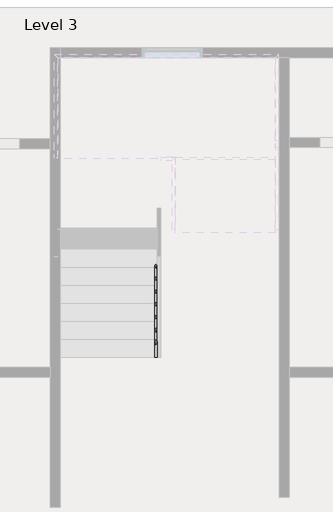
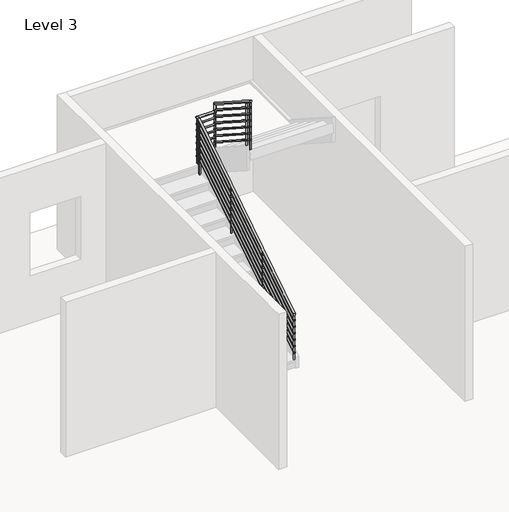
# One storey, part 6 of 7: 1 railing.
"""IFC4 building model written with IfcOpenShell, lengths in millimetres."""

from ifc_helpers import new_model, si_unit, point, frame, frame_2d, origin, place, context, project, spatial, circle_curve, ellipse_curve, trimmed, segment, composite_curve, outline, extrude, element, save
from ifc_brep_helpers import plane_surface, cylinder_surface, advanced_brep

model = new_model("IFC4")

# Units and contexts
model_context = context("Model", 3, world=origin())
ifc_project = project(units=[si_unit("LENGTHUNIT", "METRE", prefix="MILLI")], contexts=[model_context])

# Site, building, storey
site = spatial("IfcSite", under=ifc_project)
building = spatial("IfcBuilding", under=site)
storey = spatial("IfcBuildingStorey", under=building, Name="Level 3", Elevation=6500.0)

# Railing
placement = place(None, origin())
element("IfcRailing", 1, ObjectType="900mm Pipe", at=placement, inside=storey, context=model_context, shape_type="SolidModel", body=[
    advanced_brep(
    [(-504.8393676, 4284.7509075, 7552.7068065), (-544.8393676, 4284.7509075, 7552.7068065), (-504.8393676, 7315.616134, 9497.6470588), (-544.8393676, 7315.616134, 9497.6470588), (-504.8393676, 7337.8781803, 9497.6470588), (-544.8393676, 7377.8781803, 9497.6470588), (-201.3120949, 7337.8781803, 9497.6470588), (-201.3120949, 7377.8781803, 9497.6470588)],
    [
        (0, 1, ellipse_curve(frame((-524.8393676, 4284.7509075, 7552.7068065), z_axis=(0.0, -1.0, 0.0), x_axis=(0.0, 0.0, -1.0)), 23.7637817, 20.0)),
        (1, 0, ellipse_curve(frame((-524.8393676, 4284.7509075, 7552.7068065), z_axis=(0.0, -1.0, 0.0), x_axis=(0.0, 0.0, -1.0)), 23.7637817, 20.0)),
        (0, 2),
        (2, 3, ellipse_curve(frame((-524.8393676, 7315.616134, 9497.6470588), z_axis=(0.0, -0.9595876426002528, -0.28140994326585117), x_axis=(0.0, 0.28140994326585106, -0.9595876426002529)), 20.8422859, 20.0)),
        (3, 1),
        (3, 2, ellipse_curve(frame((-524.8393676, 7315.616134, 9497.6470588), z_axis=(0.0, -0.9595876426002528, -0.28140994326585117), x_axis=(0.0, 0.28140994326585106, -0.9595876426002529)), 20.8422859, 20.0)),
        (2, 4),
        (4, 5, ellipse_curve(frame((-524.8393676, 7357.8781803, 9497.6470588), z_axis=(-0.7071067811865475, -0.7071067811865475, 0.0), x_axis=(0.7071067811865474, -0.7071067811865476, 0.0)), 28.2842712, 20.0)),
        (5, 3),
        (5, 4, ellipse_curve(frame((-524.8393676, 7357.8781803, 9497.6470588), z_axis=(-0.7071067811865475, -0.7071067811865475, 0.0), x_axis=(0.7071067811865474, -0.7071067811865476, 0.0)), 28.2842712, 20.0)),
        (6, 7, ellipse_curve(frame((-201.3120949, 7357.8781803, 9497.6470588), z_axis=(0.7071067811865476, 0.0, 0.7071067811865476), x_axis=(-0.7071067811865475, 0.0, 0.7071067811865476)), 28.2842712, 20.0)),
        (7, 6, ellipse_curve(frame((-201.3120949, 7357.8781803, 9497.6470588), z_axis=(0.7071067811865476, 0.0, 0.7071067811865476), x_axis=(-0.7071067811865475, 0.0, 0.7071067811865476)), 28.2842712, 20.0)),
        (4, 6),
        (7, 5),
    ],
    [
        plane_surface(frame((-524.8393676, 4284.7509075, 7576.4705882), z_axis=(0.0, -1.0, 0.0), x_axis=(0.0, 0.0, 1.0))),
        cylinder_surface(frame((-524.8393676, 4295.5524077, 7559.6382505), z_axis=(0.0, -0.8416168876622209, -0.5400750081254979), x_axis=(-1.0, 0.0, 0.0)), 20.0),
        cylinder_surface(frame((-524.8393676, 7309.7509075, 9497.6470588), z_axis=(0.0, -1.0, 0.0), x_axis=(-1.0, 0.0, 0.0)), 20.0),
        plane_surface(frame((-221.3120949, 7357.8781803, 9517.6470588), z_axis=(0.7071067811865476, 0.0, 0.7071067811865476), x_axis=(0.7071067811865476, 0.0, -0.7071067811865476))),
        cylinder_surface(frame((-524.8393676, 7357.8781803, 9497.6470588), z_axis=(-1.0, 0.0, 0.0), x_axis=(0.0, 1.0, 0.0)), 20.0),
    ],
    [
        (0, [[1, 2]]),
        (1, [[-1, 3, 4, 5]]),
        (1, [[-2, -5, 6, -3]]),
        (2, [[-4, 7, 8, 9]]),
        (2, [[-6, -9, 10, -7]]),
        (3, [[11, 12]]),
        (4, [[-8, 13, -12, 14]]),
        (4, [[-10, -14, -11, -13]]),
    ],
),
    advanced_brep(
    [(-201.3120949, 7337.8781803, 9497.6470588), (-201.3120949, 7377.8781803, 9497.6470588), (-201.3120949, 7337.8781803, 9643.124843), (-201.3120949, 7377.8781803, 9664.9839572)],
    [
        (0, 1, ellipse_curve(frame((-201.3120949, 7357.8781803, 9497.6470588), z_axis=(-0.7071067811865476, 0.0, -0.7071067811865476), x_axis=(0.7071067811865476, 0.0, -0.7071067811865474)), 28.2842712, 20.0)),
        (1, 0, ellipse_curve(frame((-201.3120949, 7357.8781803, 9497.6470588), z_axis=(-0.7071067811865476, 0.0, -0.7071067811865476), x_axis=(0.7071067811865476, 0.0, -0.7071067811865474)), 28.2842712, 20.0)),
        (2, 3, ellipse_curve(frame((-201.3120949, 7357.8781803, 9654.0544001), z_axis=(0.0, -0.47954405004884676, 0.877517808402057), x_axis=(0.0, -0.8775178084020571, -0.47954405004884676)), 22.7915602, 20.0)),
        (3, 2, ellipse_curve(frame((-201.3120949, 7357.8781803, 9654.0544001), z_axis=(0.0, -0.47954405004884676, 0.877517808402057), x_axis=(0.0, -0.8775178084020571, -0.47954405004884676)), 22.7915602, 20.0)),
        (0, 2),
        (3, 1),
    ],
    [
        plane_surface(frame((-201.3120949, 7357.8781803, 9497.6470588), z_axis=(-0.7071067811865476, 0.0, -0.7071067811865476), x_axis=(0.7071067811865476, 0.0, -0.7071067811865476))),
        plane_surface(frame((-201.3120949, 7357.8781803, 9654.0544001), z_axis=(0.0, -0.47954405004884676, 0.877517808402057), x_axis=(1.0, 0.0, 0.0))),
        cylinder_surface(frame((-201.3120949, 7357.8781803, 9497.6470588), z_axis=(0.0, 0.0, -1.0), x_axis=(0.0, 1.0, 0.0)), 20.0),
    ],
    [
        (0, [[1, 2]]),
        (1, [[3, 4]]),
        (2, [[-1, 5, -4, 6]]),
        (2, [[-2, -6, -3, -5]]),
    ],
),
    advanced_brep(
    [(-221.3120949, 7357.8781803, 9654.0544001), (-181.3120949, 7357.8781803, 9654.0544001), (-221.3120949, 6232.4781803, 10376.2362183), (-181.3120949, 6232.4781803, 10376.2362183)],
    [
        (0, 1, ellipse_curve(frame((-201.3120949, 7357.8781803, 9654.0544001), z_axis=(0.0, 0.47954405004884676, -0.877517808402057), x_axis=(0.0, 0.8775178084020568, 0.47954405004884676)), 22.7915602, 20.0)),
        (1, 0, ellipse_curve(frame((-201.3120949, 7357.8781803, 9654.0544001), z_axis=(0.0, 0.47954405004884676, -0.877517808402057), x_axis=(0.0, 0.8775178084020568, 0.47954405004884676)), 22.7915602, 20.0)),
        (2, 3, ellipse_curve(frame((-201.3120949, 6232.4781803, 10376.2362183), z_axis=(0.0, -1.0, 0.0), x_axis=(0.0, 0.0, -1.0)), 23.7637817, 20.0)),
        (3, 2, ellipse_curve(frame((-201.3120949, 6232.4781803, 10376.2362183), z_axis=(0.0, -1.0, 0.0), x_axis=(0.0, 0.0, -1.0)), 23.7637817, 20.0)),
        (0, 2),
        (3, 1),
    ],
    [
        plane_surface(frame((-201.3120949, 7377.8781803, 9664.9839572), z_axis=(0.0, 0.47954405004884676, -0.877517808402057), x_axis=(1.0, 0.0, 0.0))),
        plane_surface(frame((-201.3120949, 6232.4781803, 10400.0), z_axis=(0.0, -1.0, 0.0), x_axis=(0.0, 0.0, -1.0))),
        cylinder_surface(frame((-201.3120949, 7367.0766801, 9648.1516195), z_axis=(0.0, 0.8416168876622208, -0.5400750081254984), x_axis=(1.0, 0.0, 0.0)), 20.0),
    ],
    [
        (0, [[1, 2]]),
        (1, [[3, 4]]),
        (2, [[-1, 5, -4, 6]]),
        (2, [[-2, -6, -3, -5]]),
    ],
),
    advanced_brep(
    [(-539.8393676, 4284.7509075, 7433.647752), (-509.8393676, 4284.7509075, 7433.647752), (-539.8393676, 7309.7509075, 9374.8242225), (-509.8393676, 7309.7509075, 9374.8242225)],
    [
        (0, 1, ellipse_curve(frame((-524.8393676, 4284.7509075, 7433.647752), z_axis=(0.0, -1.0, 0.0), x_axis=(0.0, 0.0, -1.0)), 17.8228363, 15.0)),
        (1, 0, ellipse_curve(frame((-524.8393676, 4284.7509075, 7433.647752), z_axis=(0.0, -1.0, 0.0), x_axis=(0.0, 0.0, -1.0)), 17.8228363, 15.0)),
        (2, 3, ellipse_curve(frame((-524.8393676, 7309.7509075, 9374.8242225), z_axis=(0.0, 1.0, 0.0), x_axis=(0.0, 0.0, -1.0)), 17.8228363, 15.0)),
        (3, 2, ellipse_curve(frame((-524.8393676, 7309.7509075, 9374.8242225), z_axis=(0.0, 1.0, 0.0), x_axis=(0.0, 0.0, -1.0)), 17.8228363, 15.0)),
        (0, 2),
        (3, 1),
    ],
    [
        plane_surface(frame((-524.8393676, 4284.7509075, 7451.4705882), z_axis=(0.0, -1.0, 0.0), x_axis=(0.0, 0.0, 1.0))),
        plane_surface(frame((-524.8393676, 7309.7509075, 9392.6470588), z_axis=(0.0, 1.0, 0.0), x_axis=(0.0, 0.0, 1.0))),
        cylinder_surface(frame((-524.8393676, 4292.8520327, 7438.8463349), z_axis=(0.0, -0.8416168876622209, -0.5400750081254979), x_axis=(1.0, 0.0, 0.0)), 15.0),
    ],
    [
        (0, [[1, 2]]),
        (1, [[3, 4]]),
        (2, [[-1, 5, -4, 6]]),
        (2, [[-2, -6, -3, -5]]),
    ],
),
    advanced_brep(
    [(-539.8393676, 7309.7509075, 9377.6470588), (-509.8393676, 7309.7509075, 9377.6470588), (-539.8393676, 7342.8781803, 9377.6470588), (-509.8393676, 7342.8781803, 9377.6470588)],
    [
        (0, 1, circle_curve(frame((-524.8393676, 7309.7509075, 9377.6470588), z_axis=(0.0, -1.0, 0.0), x_axis=(1.0, 0.0, 0.0)), 15.0)),
        (1, 0, circle_curve(frame((-524.8393676, 7309.7509075, 9377.6470588), z_axis=(0.0, -1.0, 0.0), x_axis=(1.0, 0.0, 0.0)), 15.0)),
        (2, 3, circle_curve(frame((-524.8393676, 7342.8781803, 9377.6470588), z_axis=(0.0, 1.0, 0.0), x_axis=(1.0, 0.0, 0.0)), 15.0)),
        (3, 2, circle_curve(frame((-524.8393676, 7342.8781803, 9377.6470588), z_axis=(0.0, 1.0, 0.0), x_axis=(1.0, 0.0, 0.0)), 15.0)),
        (0, 2),
        (3, 1),
    ],
    [
        plane_surface(frame((-524.8393676, 7309.7509075, 9392.6470588), z_axis=(0.0, -1.0, 0.0), x_axis=(0.0, 0.0, 1.0))),
        plane_surface(frame((-524.8393676, 7342.8781803, 9392.6470588), z_axis=(0.0, 1.0, 0.0), x_axis=(0.0, 0.0, 1.0))),
        cylinder_surface(frame((-524.8393676, 7309.7509075, 9377.6470588), z_axis=(0.0, -1.0, 0.0), x_axis=(1.0, 0.0, 0.0)), 15.0),
    ],
    [
        (0, [[1, 2]]),
        (1, [[3, 4]]),
        (2, [[-1, 5, -4, 6]]),
        (2, [[-2, -6, -3, -5]]),
    ],
),
    advanced_brep(
    [(-539.8393676, 7372.8781803, 9377.6470588), (-539.8393676, 7342.8781803, 9377.6470588), (-216.3120949, 7372.8781803, 9377.6470588), (-216.3120949, 7342.8781803, 9377.6470588)],
    [
        (0, 1, circle_curve(frame((-539.8393676, 7357.8781803, 9377.6470588), z_axis=(-1.0, 0.0, 0.0), x_axis=(0.0, -1.0, 0.0)), 15.0)),
        (1, 0, circle_curve(frame((-539.8393676, 7357.8781803, 9377.6470588), z_axis=(-1.0, 0.0, 0.0), x_axis=(0.0, -1.0, 0.0)), 15.0)),
        (2, 3, circle_curve(frame((-216.3120949, 7357.8781803, 9377.6470588), z_axis=(1.0, 0.0, 0.0), x_axis=(0.0, -1.0, 0.0)), 15.0)),
        (3, 2, circle_curve(frame((-216.3120949, 7357.8781803, 9377.6470588), z_axis=(1.0, 0.0, 0.0), x_axis=(0.0, -1.0, 0.0)), 15.0)),
        (0, 2),
        (3, 1),
    ],
    [
        plane_surface(frame((-539.8393676, 7357.8781803, 9392.6470588), z_axis=(-1.0, 0.0, 0.0), x_axis=(0.0, 1.0, 0.0))),
        plane_surface(frame((-216.3120949, 7357.8781803, 9392.6470588), z_axis=(1.0, 0.0, 0.0), x_axis=(0.0, 1.0, 0.0))),
        cylinder_surface(frame((-539.8393676, 7357.8781803, 9377.6470588), z_axis=(-1.0, 0.0, 0.0), x_axis=(0.0, -1.0, 0.0)), 15.0),
    ],
    [
        (0, [[1, 2]]),
        (1, [[3, 4]]),
        (2, [[-1, 5, -4, 6]]),
        (2, [[-2, -6, -3, -5]]),
    ],
),
    advanced_brep(
    [(-186.3120949, 7372.8781803, 9525.3696771), (-216.3120949, 7372.8781803, 9525.3696771), (-186.3120949, 6232.4781803, 10257.1771637), (-216.3120949, 6232.4781803, 10257.1771637)],
    [
        (0, 1, ellipse_curve(frame((-201.3120949, 7372.8781803, 9525.3696771), z_axis=(0.0, 1.0, 0.0), x_axis=(0.0, 0.0, -1.0)), 17.8228363, 15.0)),
        (1, 0, ellipse_curve(frame((-201.3120949, 7372.8781803, 9525.3696771), z_axis=(0.0, 1.0, 0.0), x_axis=(0.0, 0.0, -1.0)), 17.8228363, 15.0)),
        (2, 3, ellipse_curve(frame((-201.3120949, 6232.4781803, 10257.1771637), z_axis=(0.0, -1.0, 0.0), x_axis=(0.0, 0.0, -1.0)), 17.8228363, 15.0)),
        (3, 2, ellipse_curve(frame((-201.3120949, 6232.4781803, 10257.1771637), z_axis=(0.0, -1.0, 0.0), x_axis=(0.0, 0.0, -1.0)), 17.8228363, 15.0)),
        (0, 2),
        (3, 1),
    ],
    [
        plane_surface(frame((-201.3120949, 7372.8781803, 9543.1925134), z_axis=(0.0, 1.0, 0.0), x_axis=(0.0, 0.0, -1.0))),
        plane_surface(frame((-201.3120949, 6232.4781803, 10275.0), z_axis=(0.0, -1.0, 0.0), x_axis=(0.0, 0.0, -1.0))),
        cylinder_surface(frame((-201.3120949, 7364.7770552, 9530.5682601), z_axis=(0.0, 0.8416168876622208, -0.5400750081254984), x_axis=(-1.0, 0.0, 0.0)), 15.0),
    ],
    [
        (0, [[1, 2]]),
        (1, [[3, 4]]),
        (2, [[-1, 5, -4, 6]]),
        (2, [[-2, -6, -3, -5]]),
    ],
),
    advanced_brep(
    [(-539.8393676, 4284.7509075, 7308.647752), (-509.8393676, 4284.7509075, 7308.647752), (-539.8393676, 7309.7509075, 9249.8242225), (-509.8393676, 7309.7509075, 9249.8242225)],
    [
        (0, 1, ellipse_curve(frame((-524.8393676, 4284.7509075, 7308.647752), z_axis=(0.0, -1.0, 0.0), x_axis=(0.0, 0.0, -1.0)), 17.8228363, 15.0)),
        (1, 0, ellipse_curve(frame((-524.8393676, 4284.7509075, 7308.647752), z_axis=(0.0, -1.0, 0.0), x_axis=(0.0, 0.0, -1.0)), 17.8228363, 15.0)),
        (2, 3, ellipse_curve(frame((-524.8393676, 7309.7509075, 9249.8242225), z_axis=(0.0, 1.0, 0.0), x_axis=(0.0, 0.0, -1.0)), 17.8228363, 15.0)),
        (3, 2, ellipse_curve(frame((-524.8393676, 7309.7509075, 9249.8242225), z_axis=(0.0, 1.0, 0.0), x_axis=(0.0, 0.0, -1.0)), 17.8228363, 15.0)),
        (0, 2),
        (3, 1),
    ],
    [
        plane_surface(frame((-524.8393676, 4284.7509075, 7326.4705882), z_axis=(0.0, -1.0, 0.0), x_axis=(0.0, 0.0, 1.0))),
        plane_surface(frame((-524.8393676, 7309.7509075, 9267.6470588), z_axis=(0.0, 1.0, 0.0), x_axis=(0.0, 0.0, 1.0))),
        cylinder_surface(frame((-524.8393676, 4292.8520327, 7313.8463349), z_axis=(0.0, -0.8416168876622209, -0.5400750081254979), x_axis=(1.0, 0.0, 0.0)), 15.0),
    ],
    [
        (0, [[1, 2]]),
        (1, [[3, 4]]),
        (2, [[-1, 5, -4, 6]]),
        (2, [[-2, -6, -3, -5]]),
    ],
),
    advanced_brep(
    [(-539.8393676, 7309.7509075, 9252.6470588), (-509.8393676, 7309.7509075, 9252.6470588), (-539.8393676, 7342.8781803, 9252.6470588), (-509.8393676, 7342.8781803, 9252.6470588)],
    [
        (0, 1, circle_curve(frame((-524.8393676, 7309.7509075, 9252.6470588), z_axis=(0.0, -1.0, 0.0), x_axis=(1.0, 0.0, 0.0)), 15.0)),
        (1, 0, circle_curve(frame((-524.8393676, 7309.7509075, 9252.6470588), z_axis=(0.0, -1.0, 0.0), x_axis=(1.0, 0.0, 0.0)), 15.0)),
        (2, 3, circle_curve(frame((-524.8393676, 7342.8781803, 9252.6470588), z_axis=(0.0, 1.0, 0.0), x_axis=(1.0, 0.0, 0.0)), 15.0)),
        (3, 2, circle_curve(frame((-524.8393676, 7342.8781803, 9252.6470588), z_axis=(0.0, 1.0, 0.0), x_axis=(1.0, 0.0, 0.0)), 15.0)),
        (0, 2),
        (3, 1),
    ],
    [
        plane_surface(frame((-524.8393676, 7309.7509075, 9267.6470588), z_axis=(0.0, -1.0, 0.0), x_axis=(0.0, 0.0, 1.0))),
        plane_surface(frame((-524.8393676, 7342.8781803, 9267.6470588), z_axis=(0.0, 1.0, 0.0), x_axis=(0.0, 0.0, 1.0))),
        cylinder_surface(frame((-524.8393676, 7309.7509075, 9252.6470588), z_axis=(0.0, -1.0, 0.0), x_axis=(1.0, 0.0, 0.0)), 15.0),
    ],
    [
        (0, [[1, 2]]),
        (1, [[3, 4]]),
        (2, [[-1, 5, -4, 6]]),
        (2, [[-2, -6, -3, -5]]),
    ],
),
    advanced_brep(
    [(-539.8393676, 7372.8781803, 9252.6470588), (-539.8393676, 7342.8781803, 9252.6470588), (-216.3120949, 7372.8781803, 9252.6470588), (-216.3120949, 7342.8781803, 9252.6470588)],
    [
        (0, 1, circle_curve(frame((-539.8393676, 7357.8781803, 9252.6470588), z_axis=(-1.0, 0.0, 0.0), x_axis=(0.0, -1.0, 0.0)), 15.0)),
        (1, 0, circle_curve(frame((-539.8393676, 7357.8781803, 9252.6470588), z_axis=(-1.0, 0.0, 0.0), x_axis=(0.0, -1.0, 0.0)), 15.0)),
        (2, 3, circle_curve(frame((-216.3120949, 7357.8781803, 9252.6470588), z_axis=(1.0, 0.0, 0.0), x_axis=(0.0, -1.0, 0.0)), 15.0)),
        (3, 2, circle_curve(frame((-216.3120949, 7357.8781803, 9252.6470588), z_axis=(1.0, 0.0, 0.0), x_axis=(0.0, -1.0, 0.0)), 15.0)),
        (0, 2),
        (3, 1),
    ],
    [
        plane_surface(frame((-539.8393676, 7357.8781803, 9267.6470588), z_axis=(-1.0, 0.0, 0.0), x_axis=(0.0, 1.0, 0.0))),
        plane_surface(frame((-216.3120949, 7357.8781803, 9267.6470588), z_axis=(1.0, 0.0, 0.0), x_axis=(0.0, 1.0, 0.0))),
        cylinder_surface(frame((-539.8393676, 7357.8781803, 9252.6470588), z_axis=(-1.0, 0.0, 0.0), x_axis=(0.0, -1.0, 0.0)), 15.0),
    ],
    [
        (0, [[1, 2]]),
        (1, [[3, 4]]),
        (2, [[-1, 5, -4, 6]]),
        (2, [[-2, -6, -3, -5]]),
    ],
),
    advanced_brep(
    [(-186.3120949, 7372.8781803, 9400.3696771), (-216.3120949, 7372.8781803, 9400.3696771), (-186.3120949, 6232.4781803, 10132.1771637), (-216.3120949, 6232.4781803, 10132.1771637)],
    [
        (0, 1, ellipse_curve(frame((-201.3120949, 7372.8781803, 9400.3696771), z_axis=(0.0, 1.0, 0.0), x_axis=(0.0, 0.0, -1.0)), 17.8228363, 15.0)),
        (1, 0, ellipse_curve(frame((-201.3120949, 7372.8781803, 9400.3696771), z_axis=(0.0, 1.0, 0.0), x_axis=(0.0, 0.0, -1.0)), 17.8228363, 15.0)),
        (2, 3, ellipse_curve(frame((-201.3120949, 6232.4781803, 10132.1771637), z_axis=(0.0, -1.0, 0.0), x_axis=(0.0, 0.0, -1.0)), 17.8228363, 15.0)),
        (3, 2, ellipse_curve(frame((-201.3120949, 6232.4781803, 10132.1771637), z_axis=(0.0, -1.0, 0.0), x_axis=(0.0, 0.0, -1.0)), 17.8228363, 15.0)),
        (0, 2),
        (3, 1),
    ],
    [
        plane_surface(frame((-201.3120949, 7372.8781803, 9418.1925134), z_axis=(0.0, 1.0, 0.0), x_axis=(0.0, 0.0, -1.0))),
        plane_surface(frame((-201.3120949, 6232.4781803, 10150.0), z_axis=(0.0, -1.0, 0.0), x_axis=(0.0, 0.0, -1.0))),
        cylinder_surface(frame((-201.3120949, 7364.7770552, 9405.5682601), z_axis=(0.0, 0.8416168876622208, -0.5400750081254984), x_axis=(-1.0, 0.0, 0.0)), 15.0),
    ],
    [
        (0, [[1, 2]]),
        (1, [[3, 4]]),
        (2, [[-1, 5, -4, 6]]),
        (2, [[-2, -6, -3, -5]]),
    ],
),
    advanced_brep(
    [(-539.8393676, 4284.7509075, 7183.647752), (-509.8393676, 4284.7509075, 7183.647752), (-539.8393676, 7309.7509075, 9124.8242225), (-509.8393676, 7309.7509075, 9124.8242225)],
    [
        (0, 1, ellipse_curve(frame((-524.8393676, 4284.7509075, 7183.647752), z_axis=(0.0, -1.0, 0.0), x_axis=(0.0, 0.0, -1.0)), 17.8228363, 15.0)),
        (1, 0, ellipse_curve(frame((-524.8393676, 4284.7509075, 7183.647752), z_axis=(0.0, -1.0, 0.0), x_axis=(0.0, 0.0, -1.0)), 17.8228363, 15.0)),
        (2, 3, ellipse_curve(frame((-524.8393676, 7309.7509075, 9124.8242225), z_axis=(0.0, 1.0, 0.0), x_axis=(0.0, 0.0, -1.0)), 17.8228363, 15.0)),
        (3, 2, ellipse_curve(frame((-524.8393676, 7309.7509075, 9124.8242225), z_axis=(0.0, 1.0, 0.0), x_axis=(0.0, 0.0, -1.0)), 17.8228363, 15.0)),
        (0, 2),
        (3, 1),
    ],
    [
        plane_surface(frame((-524.8393676, 4284.7509075, 7201.4705882), z_axis=(0.0, -1.0, 0.0), x_axis=(0.0, 0.0, 1.0))),
        plane_surface(frame((-524.8393676, 7309.7509075, 9142.6470588), z_axis=(0.0, 1.0, 0.0), x_axis=(0.0, 0.0, 1.0))),
        cylinder_surface(frame((-524.8393676, 4292.8520327, 7188.8463349), z_axis=(0.0, -0.8416168876622209, -0.5400750081254979), x_axis=(1.0, 0.0, 0.0)), 15.0),
    ],
    [
        (0, [[1, 2]]),
        (1, [[3, 4]]),
        (2, [[-1, 5, -4, 6]]),
        (2, [[-2, -6, -3, -5]]),
    ],
),
    advanced_brep(
    [(-539.8393676, 7309.7509075, 9127.6470588), (-509.8393676, 7309.7509075, 9127.6470588), (-539.8393676, 7342.8781803, 9127.6470588), (-509.8393676, 7342.8781803, 9127.6470588)],
    [
        (0, 1, circle_curve(frame((-524.8393676, 7309.7509075, 9127.6470588), z_axis=(0.0, -1.0, 0.0), x_axis=(1.0, 0.0, 0.0)), 15.0)),
        (1, 0, circle_curve(frame((-524.8393676, 7309.7509075, 9127.6470588), z_axis=(0.0, -1.0, 0.0), x_axis=(1.0, 0.0, 0.0)), 15.0)),
        (2, 3, circle_curve(frame((-524.8393676, 7342.8781803, 9127.6470588), z_axis=(0.0, 1.0, 0.0), x_axis=(1.0, 0.0, 0.0)), 15.0)),
        (3, 2, circle_curve(frame((-524.8393676, 7342.8781803, 9127.6470588), z_axis=(0.0, 1.0, 0.0), x_axis=(1.0, 0.0, 0.0)), 15.0)),
        (0, 2),
        (3, 1),
    ],
    [
        plane_surface(frame((-524.8393676, 7309.7509075, 9142.6470588), z_axis=(0.0, -1.0, 0.0), x_axis=(0.0, 0.0, 1.0))),
        plane_surface(frame((-524.8393676, 7342.8781803, 9142.6470588), z_axis=(0.0, 1.0, 0.0), x_axis=(0.0, 0.0, 1.0))),
        cylinder_surface(frame((-524.8393676, 7309.7509075, 9127.6470588), z_axis=(0.0, -1.0, 0.0), x_axis=(1.0, 0.0, 0.0)), 15.0),
    ],
    [
        (0, [[1, 2]]),
        (1, [[3, 4]]),
        (2, [[-1, 5, -4, 6]]),
        (2, [[-2, -6, -3, -5]]),
    ],
),
    advanced_brep(
    [(-539.8393676, 7372.8781803, 9127.6470588), (-539.8393676, 7342.8781803, 9127.6470588), (-216.3120949, 7372.8781803, 9127.6470588), (-216.3120949, 7342.8781803, 9127.6470588)],
    [
        (0, 1, circle_curve(frame((-539.8393676, 7357.8781803, 9127.6470588), z_axis=(-1.0, 0.0, 0.0), x_axis=(0.0, -1.0, 0.0)), 15.0)),
        (1, 0, circle_curve(frame((-539.8393676, 7357.8781803, 9127.6470588), z_axis=(-1.0, 0.0, 0.0), x_axis=(0.0, -1.0, 0.0)), 15.0)),
        (2, 3, circle_curve(frame((-216.3120949, 7357.8781803, 9127.6470588), z_axis=(1.0, 0.0, 0.0), x_axis=(0.0, -1.0, 0.0)), 15.0)),
        (3, 2, circle_curve(frame((-216.3120949, 7357.8781803, 9127.6470588), z_axis=(1.0, 0.0, 0.0), x_axis=(0.0, -1.0, 0.0)), 15.0)),
        (0, 2),
        (3, 1),
    ],
    [
        plane_surface(frame((-539.8393676, 7357.8781803, 9142.6470588), z_axis=(-1.0, 0.0, 0.0), x_axis=(0.0, 1.0, 0.0))),
        plane_surface(frame((-216.3120949, 7357.8781803, 9142.6470588), z_axis=(1.0, 0.0, 0.0), x_axis=(0.0, 1.0, 0.0))),
        cylinder_surface(frame((-539.8393676, 7357.8781803, 9127.6470588), z_axis=(-1.0, 0.0, 0.0), x_axis=(0.0, -1.0, 0.0)), 15.0),
    ],
    [
        (0, [[1, 2]]),
        (1, [[3, 4]]),
        (2, [[-1, 5, -4, 6]]),
        (2, [[-2, -6, -3, -5]]),
    ],
),
    advanced_brep(
    [(-186.3120949, 7372.8781803, 9275.3696771), (-216.3120949, 7372.8781803, 9275.3696771), (-186.3120949, 6232.4781803, 10007.1771637), (-216.3120949, 6232.4781803, 10007.1771637)],
    [
        (0, 1, ellipse_curve(frame((-201.3120949, 7372.8781803, 9275.3696771), z_axis=(0.0, 1.0, 0.0), x_axis=(0.0, 0.0, -1.0)), 17.8228363, 15.0)),
        (1, 0, ellipse_curve(frame((-201.3120949, 7372.8781803, 9275.3696771), z_axis=(0.0, 1.0, 0.0), x_axis=(0.0, 0.0, -1.0)), 17.8228363, 15.0)),
        (2, 3, ellipse_curve(frame((-201.3120949, 6232.4781803, 10007.1771637), z_axis=(0.0, -1.0, 0.0), x_axis=(0.0, 0.0, -1.0)), 17.8228363, 15.0)),
        (3, 2, ellipse_curve(frame((-201.3120949, 6232.4781803, 10007.1771637), z_axis=(0.0, -1.0, 0.0), x_axis=(0.0, 0.0, -1.0)), 17.8228363, 15.0)),
        (0, 2),
        (3, 1),
    ],
    [
        plane_surface(frame((-201.3120949, 7372.8781803, 9293.1925134), z_axis=(0.0, 1.0, 0.0), x_axis=(0.0, 0.0, -1.0))),
        plane_surface(frame((-201.3120949, 6232.4781803, 10025.0), z_axis=(0.0, -1.0, 0.0), x_axis=(0.0, 0.0, -1.0))),
        cylinder_surface(frame((-201.3120949, 7364.7770552, 9280.5682601), z_axis=(0.0, 0.8416168876622208, -0.5400750081254984), x_axis=(-1.0, 0.0, 0.0)), 15.0),
    ],
    [
        (0, [[1, 2]]),
        (1, [[3, 4]]),
        (2, [[-1, 5, -4, 6]]),
        (2, [[-2, -6, -3, -5]]),
    ],
),
    advanced_brep(
    [(-539.8393676, 4284.7509075, 7058.647752), (-509.8393676, 4284.7509075, 7058.647752), (-539.8393676, 7309.7509075, 8999.8242225), (-509.8393676, 7309.7509075, 8999.8242225)],
    [
        (0, 1, ellipse_curve(frame((-524.8393676, 4284.7509075, 7058.647752), z_axis=(0.0, -1.0, 0.0), x_axis=(0.0, 0.0, -1.0)), 17.8228363, 15.0)),
        (1, 0, ellipse_curve(frame((-524.8393676, 4284.7509075, 7058.647752), z_axis=(0.0, -1.0, 0.0), x_axis=(0.0, 0.0, -1.0)), 17.8228363, 15.0)),
        (2, 3, ellipse_curve(frame((-524.8393676, 7309.7509075, 8999.8242225), z_axis=(0.0, 1.0, 0.0), x_axis=(0.0, 0.0, -1.0)), 17.8228363, 15.0)),
        (3, 2, ellipse_curve(frame((-524.8393676, 7309.7509075, 8999.8242225), z_axis=(0.0, 1.0, 0.0), x_axis=(0.0, 0.0, -1.0)), 17.8228363, 15.0)),
        (0, 2),
        (3, 1),
    ],
    [
        plane_surface(frame((-524.8393676, 4284.7509075, 7076.4705882), z_axis=(0.0, -1.0, 0.0), x_axis=(0.0, 0.0, 1.0))),
        plane_surface(frame((-524.8393676, 7309.7509075, 9017.6470588), z_axis=(0.0, 1.0, 0.0), x_axis=(0.0, 0.0, 1.0))),
        cylinder_surface(frame((-524.8393676, 4292.8520327, 7063.8463349), z_axis=(0.0, -0.8416168876622209, -0.5400750081254979), x_axis=(1.0, 0.0, 0.0)), 15.0),
    ],
    [
        (0, [[1, 2]]),
        (1, [[3, 4]]),
        (2, [[-1, 5, -4, 6]]),
        (2, [[-2, -6, -3, -5]]),
    ],
),
    advanced_brep(
    [(-539.8393676, 7309.7509075, 9002.6470588), (-509.8393676, 7309.7509075, 9002.6470588), (-539.8393676, 7342.8781803, 9002.6470588), (-509.8393676, 7342.8781803, 9002.6470588)],
    [
        (0, 1, circle_curve(frame((-524.8393676, 7309.7509075, 9002.6470588), z_axis=(0.0, -1.0, 0.0), x_axis=(1.0, 0.0, 0.0)), 15.0)),
        (1, 0, circle_curve(frame((-524.8393676, 7309.7509075, 9002.6470588), z_axis=(0.0, -1.0, 0.0), x_axis=(1.0, 0.0, 0.0)), 15.0)),
        (2, 3, circle_curve(frame((-524.8393676, 7342.8781803, 9002.6470588), z_axis=(0.0, 1.0, 0.0), x_axis=(1.0, 0.0, 0.0)), 15.0)),
        (3, 2, circle_curve(frame((-524.8393676, 7342.8781803, 9002.6470588), z_axis=(0.0, 1.0, 0.0), x_axis=(1.0, 0.0, 0.0)), 15.0)),
        (0, 2),
        (3, 1),
    ],
    [
        plane_surface(frame((-524.8393676, 7309.7509075, 9017.6470588), z_axis=(0.0, -1.0, 0.0), x_axis=(0.0, 0.0, 1.0))),
        plane_surface(frame((-524.8393676, 7342.8781803, 9017.6470588), z_axis=(0.0, 1.0, 0.0), x_axis=(0.0, 0.0, 1.0))),
        cylinder_surface(frame((-524.8393676, 7309.7509075, 9002.6470588), z_axis=(0.0, -1.0, 0.0), x_axis=(1.0, 0.0, 0.0)), 15.0),
    ],
    [
        (0, [[1, 2]]),
        (1, [[3, 4]]),
        (2, [[-1, 5, -4, 6]]),
        (2, [[-2, -6, -3, -5]]),
    ],
),
    advanced_brep(
    [(-539.8393676, 7372.8781803, 9002.6470588), (-539.8393676, 7342.8781803, 9002.6470588), (-216.3120949, 7372.8781803, 9002.6470588), (-216.3120949, 7342.8781803, 9002.6470588)],
    [
        (0, 1, circle_curve(frame((-539.8393676, 7357.8781803, 9002.6470588), z_axis=(-1.0, 0.0, 0.0), x_axis=(0.0, -1.0, 0.0)), 15.0)),
        (1, 0, circle_curve(frame((-539.8393676, 7357.8781803, 9002.6470588), z_axis=(-1.0, 0.0, 0.0), x_axis=(0.0, -1.0, 0.0)), 15.0)),
        (2, 3, circle_curve(frame((-216.3120949, 7357.8781803, 9002.6470588), z_axis=(1.0, 0.0, 0.0), x_axis=(0.0, -1.0, 0.0)), 15.0)),
        (3, 2, circle_curve(frame((-216.3120949, 7357.8781803, 9002.6470588), z_axis=(1.0, 0.0, 0.0), x_axis=(0.0, -1.0, 0.0)), 15.0)),
        (0, 2),
        (3, 1),
    ],
    [
        plane_surface(frame((-539.8393676, 7357.8781803, 9017.6470588), z_axis=(-1.0, 0.0, 0.0), x_axis=(0.0, 1.0, 0.0))),
        plane_surface(frame((-216.3120949, 7357.8781803, 9017.6470588), z_axis=(1.0, 0.0, 0.0), x_axis=(0.0, 1.0, 0.0))),
        cylinder_surface(frame((-539.8393676, 7357.8781803, 9002.6470588), z_axis=(-1.0, 0.0, 0.0), x_axis=(0.0, -1.0, 0.0)), 15.0),
    ],
    [
        (0, [[1, 2]]),
        (1, [[3, 4]]),
        (2, [[-1, 5, -4, 6]]),
        (2, [[-2, -6, -3, -5]]),
    ],
),
    advanced_brep(
    [(-186.3120949, 7372.8781803, 9150.3696771), (-216.3120949, 7372.8781803, 9150.3696771), (-186.3120949, 6232.4781803, 9882.1771637), (-216.3120949, 6232.4781803, 9882.1771637)],
    [
        (0, 1, ellipse_curve(frame((-201.3120949, 7372.8781803, 9150.3696771), z_axis=(0.0, 1.0, 0.0), x_axis=(0.0, 0.0, -1.0)), 17.8228363, 15.0)),
        (1, 0, ellipse_curve(frame((-201.3120949, 7372.8781803, 9150.3696771), z_axis=(0.0, 1.0, 0.0), x_axis=(0.0, 0.0, -1.0)), 17.8228363, 15.0)),
        (2, 3, ellipse_curve(frame((-201.3120949, 6232.4781803, 9882.1771637), z_axis=(0.0, -1.0, 0.0), x_axis=(0.0, 0.0, -1.0)), 17.8228363, 15.0)),
        (3, 2, ellipse_curve(frame((-201.3120949, 6232.4781803, 9882.1771637), z_axis=(0.0, -1.0, 0.0), x_axis=(0.0, 0.0, -1.0)), 17.8228363, 15.0)),
        (0, 2),
        (3, 1),
    ],
    [
        plane_surface(frame((-201.3120949, 7372.8781803, 9168.1925134), z_axis=(0.0, 1.0, 0.0), x_axis=(0.0, 0.0, -1.0))),
        plane_surface(frame((-201.3120949, 6232.4781803, 9900.0), z_axis=(0.0, -1.0, 0.0), x_axis=(0.0, 0.0, -1.0))),
        cylinder_surface(frame((-201.3120949, 7364.7770552, 9155.5682601), z_axis=(0.0, 0.8416168876622208, -0.5400750081254984), x_axis=(-1.0, 0.0, 0.0)), 15.0),
    ],
    [
        (0, [[1, 2]]),
        (1, [[3, 4]]),
        (2, [[-1, 5, -4, 6]]),
        (2, [[-2, -6, -3, -5]]),
    ],
),
    advanced_brep(
    [(-539.8393676, 4284.7509075, 6933.647752), (-509.8393676, 4284.7509075, 6933.647752), (-539.8393676, 7309.7509075, 8874.8242225), (-509.8393676, 7309.7509075, 8874.8242225)],
    [
        (0, 1, ellipse_curve(frame((-524.8393676, 4284.7509075, 6933.647752), z_axis=(0.0, -1.0, 0.0), x_axis=(0.0, 0.0, -1.0)), 17.8228363, 15.0)),
        (1, 0, ellipse_curve(frame((-524.8393676, 4284.7509075, 6933.647752), z_axis=(0.0, -1.0, 0.0), x_axis=(0.0, 0.0, -1.0)), 17.8228363, 15.0)),
        (2, 3, ellipse_curve(frame((-524.8393676, 7309.7509075, 8874.8242225), z_axis=(0.0, 1.0, 0.0), x_axis=(0.0, 0.0, -1.0)), 17.8228363, 15.0)),
        (3, 2, ellipse_curve(frame((-524.8393676, 7309.7509075, 8874.8242225), z_axis=(0.0, 1.0, 0.0), x_axis=(0.0, 0.0, -1.0)), 17.8228363, 15.0)),
        (0, 2),
        (3, 1),
    ],
    [
        plane_surface(frame((-524.8393676, 4284.7509075, 6951.4705882), z_axis=(0.0, -1.0, 0.0), x_axis=(0.0, 0.0, 1.0))),
        plane_surface(frame((-524.8393676, 7309.7509075, 8892.6470588), z_axis=(0.0, 1.0, 0.0), x_axis=(0.0, 0.0, 1.0))),
        cylinder_surface(frame((-524.8393676, 4292.8520327, 6938.8463349), z_axis=(0.0, -0.8416168876622209, -0.5400750081254979), x_axis=(1.0, 0.0, 0.0)), 15.0),
    ],
    [
        (0, [[1, 2]]),
        (1, [[3, 4]]),
        (2, [[-1, 5, -4, 6]]),
        (2, [[-2, -6, -3, -5]]),
    ],
),
    advanced_brep(
    [(-539.8393676, 7309.7509075, 8877.6470588), (-509.8393676, 7309.7509075, 8877.6470588), (-539.8393676, 7342.8781803, 8877.6470588), (-509.8393676, 7342.8781803, 8877.6470588)],
    [
        (0, 1, circle_curve(frame((-524.8393676, 7309.7509075, 8877.6470588), z_axis=(0.0, -1.0, 0.0), x_axis=(1.0, 0.0, 0.0)), 15.0)),
        (1, 0, circle_curve(frame((-524.8393676, 7309.7509075, 8877.6470588), z_axis=(0.0, -1.0, 0.0), x_axis=(1.0, 0.0, 0.0)), 15.0)),
        (2, 3, circle_curve(frame((-524.8393676, 7342.8781803, 8877.6470588), z_axis=(0.0, 1.0, 0.0), x_axis=(1.0, 0.0, 0.0)), 15.0)),
        (3, 2, circle_curve(frame((-524.8393676, 7342.8781803, 8877.6470588), z_axis=(0.0, 1.0, 0.0), x_axis=(1.0, 0.0, 0.0)), 15.0)),
        (0, 2),
        (3, 1),
    ],
    [
        plane_surface(frame((-524.8393676, 7309.7509075, 8892.6470588), z_axis=(0.0, -1.0, 0.0), x_axis=(0.0, 0.0, 1.0))),
        plane_surface(frame((-524.8393676, 7342.8781803, 8892.6470588), z_axis=(0.0, 1.0, 0.0), x_axis=(0.0, 0.0, 1.0))),
        cylinder_surface(frame((-524.8393676, 7309.7509075, 8877.6470588), z_axis=(0.0, -1.0, 0.0), x_axis=(1.0, 0.0, 0.0)), 15.0),
    ],
    [
        (0, [[1, 2]]),
        (1, [[3, 4]]),
        (2, [[-1, 5, -4, 6]]),
        (2, [[-2, -6, -3, -5]]),
    ],
),
    advanced_brep(
    [(-539.8393676, 7372.8781803, 8877.6470588), (-539.8393676, 7342.8781803, 8877.6470588), (-216.3120949, 7372.8781803, 8877.6470588), (-216.3120949, 7342.8781803, 8877.6470588)],
    [
        (0, 1, circle_curve(frame((-539.8393676, 7357.8781803, 8877.6470588), z_axis=(-1.0, 0.0, 0.0), x_axis=(0.0, -1.0, 0.0)), 15.0)),
        (1, 0, circle_curve(frame((-539.8393676, 7357.8781803, 8877.6470588), z_axis=(-1.0, 0.0, 0.0), x_axis=(0.0, -1.0, 0.0)), 15.0)),
        (2, 3, circle_curve(frame((-216.3120949, 7357.8781803, 8877.6470588), z_axis=(1.0, 0.0, 0.0), x_axis=(0.0, -1.0, 0.0)), 15.0)),
        (3, 2, circle_curve(frame((-216.3120949, 7357.8781803, 8877.6470588), z_axis=(1.0, 0.0, 0.0), x_axis=(0.0, -1.0, 0.0)), 15.0)),
        (0, 2),
        (3, 1),
    ],
    [
        plane_surface(frame((-539.8393676, 7357.8781803, 8892.6470588), z_axis=(-1.0, 0.0, 0.0), x_axis=(0.0, 1.0, 0.0))),
        plane_surface(frame((-216.3120949, 7357.8781803, 8892.6470588), z_axis=(1.0, 0.0, 0.0), x_axis=(0.0, 1.0, 0.0))),
        cylinder_surface(frame((-539.8393676, 7357.8781803, 8877.6470588), z_axis=(-1.0, 0.0, 0.0), x_axis=(0.0, -1.0, 0.0)), 15.0),
    ],
    [
        (0, [[1, 2]]),
        (1, [[3, 4]]),
        (2, [[-1, 5, -4, 6]]),
        (2, [[-2, -6, -3, -5]]),
    ],
),
    advanced_brep(
    [(-186.3120949, 7372.8781803, 9025.3696771), (-216.3120949, 7372.8781803, 9025.3696771), (-186.3120949, 6232.4781803, 9757.1771637), (-216.3120949, 6232.4781803, 9757.1771637)],
    [
        (0, 1, ellipse_curve(frame((-201.3120949, 7372.8781803, 9025.3696771), z_axis=(0.0, 1.0, 0.0), x_axis=(0.0, 0.0, -1.0)), 17.8228363, 15.0)),
        (1, 0, ellipse_curve(frame((-201.3120949, 7372.8781803, 9025.3696771), z_axis=(0.0, 1.0, 0.0), x_axis=(0.0, 0.0, -1.0)), 17.8228363, 15.0)),
        (2, 3, ellipse_curve(frame((-201.3120949, 6232.4781803, 9757.1771637), z_axis=(0.0, -1.0, 0.0), x_axis=(0.0, 0.0, -1.0)), 17.8228363, 15.0)),
        (3, 2, ellipse_curve(frame((-201.3120949, 6232.4781803, 9757.1771637), z_axis=(0.0, -1.0, 0.0), x_axis=(0.0, 0.0, -1.0)), 17.8228363, 15.0)),
        (0, 2),
        (3, 1),
    ],
    [
        plane_surface(frame((-201.3120949, 7372.8781803, 9043.1925134), z_axis=(0.0, 1.0, 0.0), x_axis=(0.0, 0.0, -1.0))),
        plane_surface(frame((-201.3120949, 6232.4781803, 9775.0), z_axis=(0.0, -1.0, 0.0), x_axis=(0.0, 0.0, -1.0))),
        cylinder_surface(frame((-201.3120949, 7364.7770552, 9030.5682601), z_axis=(0.0, 0.8416168876622208, -0.5400750081254984), x_axis=(-1.0, 0.0, 0.0)), 15.0),
    ],
    [
        (0, [[1, 2]]),
        (1, [[3, 4]]),
        (2, [[-1, 5, -4, 6]]),
        (2, [[-2, -6, -3, -5]]),
    ],
),
    advanced_brep(
    [(-539.8393676, 4284.7509075, 6808.647752), (-509.8393676, 4284.7509075, 6808.647752), (-539.8393676, 7309.7509075, 8749.8242225), (-509.8393676, 7309.7509075, 8749.8242225)],
    [
        (0, 1, ellipse_curve(frame((-524.8393676, 4284.7509075, 6808.647752), z_axis=(0.0, -1.0, 0.0), x_axis=(0.0, 0.0, -1.0)), 17.8228363, 15.0)),
        (1, 0, ellipse_curve(frame((-524.8393676, 4284.7509075, 6808.647752), z_axis=(0.0, -1.0, 0.0), x_axis=(0.0, 0.0, -1.0)), 17.8228363, 15.0)),
        (2, 3, ellipse_curve(frame((-524.8393676, 7309.7509075, 8749.8242225), z_axis=(0.0, 1.0, 0.0), x_axis=(0.0, 0.0, -1.0)), 17.8228363, 15.0)),
        (3, 2, ellipse_curve(frame((-524.8393676, 7309.7509075, 8749.8242225), z_axis=(0.0, 1.0, 0.0), x_axis=(0.0, 0.0, -1.0)), 17.8228363, 15.0)),
        (0, 2),
        (3, 1),
    ],
    [
        plane_surface(frame((-524.8393676, 4284.7509075, 6826.4705882), z_axis=(0.0, -1.0, 0.0), x_axis=(0.0, 0.0, 1.0))),
        plane_surface(frame((-524.8393676, 7309.7509075, 8767.6470588), z_axis=(0.0, 1.0, 0.0), x_axis=(0.0, 0.0, 1.0))),
        cylinder_surface(frame((-524.8393676, 4292.8520327, 6813.8463349), z_axis=(0.0, -0.8416168876622209, -0.5400750081254979), x_axis=(1.0, 0.0, 0.0)), 15.0),
    ],
    [
        (0, [[1, 2]]),
        (1, [[3, 4]]),
        (2, [[-1, 5, -4, 6]]),
        (2, [[-2, -6, -3, -5]]),
    ],
),
    advanced_brep(
    [(-539.8393676, 7309.7509075, 8752.6470588), (-509.8393676, 7309.7509075, 8752.6470588), (-539.8393676, 7342.8781803, 8752.6470588), (-509.8393676, 7342.8781803, 8752.6470588)],
    [
        (0, 1, circle_curve(frame((-524.8393676, 7309.7509075, 8752.6470588), z_axis=(0.0, -1.0, 0.0), x_axis=(1.0, 0.0, 0.0)), 15.0)),
        (1, 0, circle_curve(frame((-524.8393676, 7309.7509075, 8752.6470588), z_axis=(0.0, -1.0, 0.0), x_axis=(1.0, 0.0, 0.0)), 15.0)),
        (2, 3, circle_curve(frame((-524.8393676, 7342.8781803, 8752.6470588), z_axis=(0.0, 1.0, 0.0), x_axis=(1.0, 0.0, 0.0)), 15.0)),
        (3, 2, circle_curve(frame((-524.8393676, 7342.8781803, 8752.6470588), z_axis=(0.0, 1.0, 0.0), x_axis=(1.0, 0.0, 0.0)), 15.0)),
        (0, 2),
        (3, 1),
    ],
    [
        plane_surface(frame((-524.8393676, 7309.7509075, 8767.6470588), z_axis=(0.0, -1.0, 0.0), x_axis=(0.0, 0.0, 1.0))),
        plane_surface(frame((-524.8393676, 7342.8781803, 8767.6470588), z_axis=(0.0, 1.0, 0.0), x_axis=(0.0, 0.0, 1.0))),
        cylinder_surface(frame((-524.8393676, 7309.7509075, 8752.6470588), z_axis=(0.0, -1.0, 0.0), x_axis=(1.0, 0.0, 0.0)), 15.0),
    ],
    [
        (0, [[1, 2]]),
        (1, [[3, 4]]),
        (2, [[-1, 5, -4, 6]]),
        (2, [[-2, -6, -3, -5]]),
    ],
),
    advanced_brep(
    [(-539.8393676, 7372.8781803, 8752.6470588), (-539.8393676, 7342.8781803, 8752.6470588), (-216.3120949, 7372.8781803, 8752.6470588), (-216.3120949, 7342.8781803, 8752.6470588)],
    [
        (0, 1, circle_curve(frame((-539.8393676, 7357.8781803, 8752.6470588), z_axis=(-1.0, 0.0, 0.0), x_axis=(0.0, -1.0, 0.0)), 15.0)),
        (1, 0, circle_curve(frame((-539.8393676, 7357.8781803, 8752.6470588), z_axis=(-1.0, 0.0, 0.0), x_axis=(0.0, -1.0, 0.0)), 15.0)),
        (2, 3, circle_curve(frame((-216.3120949, 7357.8781803, 8752.6470588), z_axis=(1.0, 0.0, 0.0), x_axis=(0.0, -1.0, 0.0)), 15.0)),
        (3, 2, circle_curve(frame((-216.3120949, 7357.8781803, 8752.6470588), z_axis=(1.0, 0.0, 0.0), x_axis=(0.0, -1.0, 0.0)), 15.0)),
        (0, 2),
        (3, 1),
    ],
    [
        plane_surface(frame((-539.8393676, 7357.8781803, 8767.6470588), z_axis=(-1.0, 0.0, 0.0), x_axis=(0.0, 1.0, 0.0))),
        plane_surface(frame((-216.3120949, 7357.8781803, 8767.6470588), z_axis=(1.0, 0.0, 0.0), x_axis=(0.0, 1.0, 0.0))),
        cylinder_surface(frame((-539.8393676, 7357.8781803, 8752.6470588), z_axis=(-1.0, 0.0, 0.0), x_axis=(0.0, -1.0, 0.0)), 15.0),
    ],
    [
        (0, [[1, 2]]),
        (1, [[3, 4]]),
        (2, [[-1, 5, -4, 6]]),
        (2, [[-2, -6, -3, -5]]),
    ],
),
    advanced_brep(
    [(-186.3120949, 7372.8781803, 8900.3696771), (-216.3120949, 7372.8781803, 8900.3696771), (-186.3120949, 6232.4781803, 9632.1771637), (-216.3120949, 6232.4781803, 9632.1771637)],
    [
        (0, 1, ellipse_curve(frame((-201.3120949, 7372.8781803, 8900.3696771), z_axis=(0.0, 1.0, 0.0), x_axis=(0.0, 0.0, -1.0)), 17.8228363, 15.0)),
        (1, 0, ellipse_curve(frame((-201.3120949, 7372.8781803, 8900.3696771), z_axis=(0.0, 1.0, 0.0), x_axis=(0.0, 0.0, -1.0)), 17.8228363, 15.0)),
        (2, 3, ellipse_curve(frame((-201.3120949, 6232.4781803, 9632.1771637), z_axis=(0.0, -1.0, 0.0), x_axis=(0.0, 0.0, -1.0)), 17.8228363, 15.0)),
        (3, 2, ellipse_curve(frame((-201.3120949, 6232.4781803, 9632.1771637), z_axis=(0.0, -1.0, 0.0), x_axis=(0.0, 0.0, -1.0)), 17.8228363, 15.0)),
        (0, 2),
        (3, 1),
    ],
    [
        plane_surface(frame((-201.3120949, 7372.8781803, 8918.1925134), z_axis=(0.0, 1.0, 0.0), x_axis=(0.0, 0.0, -1.0))),
        plane_surface(frame((-201.3120949, 6232.4781803, 9650.0), z_axis=(0.0, -1.0, 0.0), x_axis=(0.0, 0.0, -1.0))),
        cylinder_surface(frame((-201.3120949, 7364.7770552, 8905.5682601), z_axis=(0.0, 0.8416168876622208, -0.5400750081254984), x_axis=(-1.0, 0.0, 0.0)), 15.0),
    ],
    [
        (0, [[1, 2]]),
        (1, [[3, 4]]),
        (2, [[-1, 5, -4, 6]]),
        (2, [[-2, -6, -3, -5]]),
    ],
),
    advanced_brep(
    [(-213.8120949, 6357.8781803, 10272.0018483), (-213.8120949, 6357.8781803, 9323.5294118), (-188.8120949, 6357.8781803, 9323.5294118), (-188.8120949, 6357.8781803, 10272.0018483)],
    [
        (0, 1),
        (1, 2, circle_curve(frame((-201.3120949, 6357.8781803, 9323.5294118), z_axis=(0.0, 0.0, 1.0), x_axis=(1.0, 0.0, 0.0)), 12.5)),
        (2, 3),
        (3, 0, ellipse_curve(frame((-201.3120949, 6357.8781803, 10272.0018483), z_axis=(0.0, -0.5400750081254972, -0.8416168876622213), x_axis=(0.0, -0.8416168876622212, 0.5400750081254974)), 14.8523636, 12.5)),
        (0, 3, ellipse_curve(frame((-201.3120949, 6357.8781803, 10272.0018483), z_axis=(0.0, -0.5400750081254972, -0.8416168876622213), x_axis=(0.0, -0.8416168876622212, 0.5400750081254974)), 14.8523636, 12.5)),
        (2, 1, circle_curve(frame((-201.3120949, 6357.8781803, 9323.5294118), z_axis=(0.0, 0.0, 1.0), x_axis=(1.0, 0.0, 0.0)), 12.5)),
    ],
    [
        cylinder_surface(frame((-201.3120949, 6357.8781803, 9223.5294118), z_axis=(0.0, 0.0, 1.0), x_axis=(1.0, 0.0, 0.0)), 12.5),
        plane_surface(frame((-176.3120949, 6332.8781803, 10288.0446291), z_axis=(0.0, 0.5400750081254972, 0.8416168876622213), x_axis=(-1.0, 0.0, 0.0))),
        plane_surface(frame((-176.3120949, 6382.8781803, 9323.5294118), z_axis=(0.0, 0.0, -1.0), x_axis=(-1.0, 0.0, 0.0))),
    ],
    [
        (0, [[1, 2, 3, 4]]),
        (0, [[-1, 5, -3, 6]]),
        (1, [[-4, -5]]),
        (2, [[-2, -6]]),
    ],
),
    advanced_brep(
    [(-512.3393676, 7284.7509075, 9454.0767147), (-512.3393676, 7284.7509075, 8441.1764706), (-537.3393676, 7284.7509075, 8441.1764706), (-537.3393676, 7284.7509075, 9454.0767147)],
    [
        (0, 1),
        (1, 2, circle_curve(frame((-524.8393676, 7284.7509075, 8441.1764706), z_axis=(0.0, 0.0, 1.0), x_axis=(-1.0, 0.0, 0.0)), 12.5)),
        (2, 3),
        (3, 0, ellipse_curve(frame((-524.8393676, 7284.7509075, 9454.0767147), z_axis=(0.0, 0.5400750081254972, -0.8416168876622212), x_axis=(0.0, 0.8416168876622212, 0.5400750081254975)), 14.8523636, 12.5)),
        (0, 3, ellipse_curve(frame((-524.8393676, 7284.7509075, 9454.0767147), z_axis=(0.0, 0.5400750081254972, -0.8416168876622212), x_axis=(0.0, 0.8416168876622212, 0.5400750081254975)), 14.8523636, 12.5)),
        (2, 1, circle_curve(frame((-524.8393676, 7284.7509075, 8441.1764706), z_axis=(0.0, 0.0, 1.0), x_axis=(-1.0, 0.0, 0.0)), 12.5)),
    ],
    [
        cylinder_surface(frame((-524.8393676, 7284.7509075, 8341.1764706), z_axis=(0.0, 0.0, 1.0), x_axis=(-1.0, 0.0, 0.0)), 12.5),
        plane_surface(frame((-549.8393676, 7309.7509075, 9470.1194954), z_axis=(0.0, -0.5400750081254972, 0.8416168876622212), x_axis=(1.0, 0.0, 0.0))),
        plane_surface(frame((-549.8393676, 7259.7509075, 8441.1764706), z_axis=(0.0, 0.0, -1.0), x_axis=(1.0, 0.0, 0.0))),
    ],
    [
        (0, [[1, 2, 3, 4]]),
        (0, [[-1, 5, -3, 6]]),
        (1, [[-4, -5]]),
        (2, [[-2, -6]]),
    ],
),
    advanced_brep(
    [(-512.3393676, 6284.7509075, 8812.3654847), (-512.3393676, 6284.7509075, 7911.7647059), (-537.3393676, 6284.7509075, 7911.7647059), (-537.3393676, 6284.7509075, 8812.3654847)],
    [
        (0, 1),
        (1, 2, circle_curve(frame((-524.8393676, 6284.7509075, 7911.7647059), z_axis=(0.0, 0.0, 1.0), x_axis=(-1.0, 0.0, 0.0)), 12.5)),
        (2, 3),
        (3, 0, ellipse_curve(frame((-524.8393676, 6284.7509075, 8812.3654847), z_axis=(0.0, 0.5400750081254972, -0.8416168876622212), x_axis=(0.0, 0.8416168876622212, 0.5400750081254975)), 14.8523636, 12.5)),
        (0, 3, ellipse_curve(frame((-524.8393676, 6284.7509075, 8812.3654847), z_axis=(0.0, 0.5400750081254972, -0.8416168876622212), x_axis=(0.0, 0.8416168876622212, 0.5400750081254975)), 14.8523636, 12.5)),
        (2, 1, circle_curve(frame((-524.8393676, 6284.7509075, 7911.7647059), z_axis=(0.0, 0.0, 1.0), x_axis=(-1.0, 0.0, 0.0)), 12.5)),
    ],
    [
        cylinder_surface(frame((-524.8393676, 6284.7509075, 7811.7647059), z_axis=(0.0, 0.0, 1.0), x_axis=(-1.0, 0.0, 0.0)), 12.5),
        plane_surface(frame((-549.8393676, 6309.7509075, 8828.4082655), z_axis=(0.0, -0.5400750081254972, 0.8416168876622212), x_axis=(1.0, 0.0, 0.0))),
        plane_surface(frame((-549.8393676, 6259.7509075, 7911.7647059), z_axis=(0.0, 0.0, -1.0), x_axis=(1.0, 0.0, 0.0))),
    ],
    [
        (0, [[1, 2, 3, 4]]),
        (0, [[-1, 5, -3, 6]]),
        (1, [[-4, -5]]),
        (2, [[-2, -6]]),
    ],
),
    advanced_brep(
    [(-512.3393676, 5284.7509075, 8170.6542548), (-512.3393676, 5284.7509075, 7205.8823529), (-537.3393676, 5284.7509075, 7205.8823529), (-537.3393676, 5284.7509075, 8170.6542548)],
    [
        (0, 1),
        (1, 2, circle_curve(frame((-524.8393676, 5284.7509075, 7205.8823529), z_axis=(0.0, 0.0, 1.0), x_axis=(-1.0, 0.0, 0.0)), 12.5)),
        (2, 3),
        (3, 0, ellipse_curve(frame((-524.8393676, 5284.7509075, 8170.6542548), z_axis=(0.0, 0.5400750081254972, -0.8416168876622212), x_axis=(0.0, 0.8416168876622212, 0.5400750081254975)), 14.8523636, 12.5)),
        (0, 3, ellipse_curve(frame((-524.8393676, 5284.7509075, 8170.6542548), z_axis=(0.0, 0.5400750081254972, -0.8416168876622212), x_axis=(0.0, 0.8416168876622212, 0.5400750081254975)), 14.8523636, 12.5)),
        (2, 1, circle_curve(frame((-524.8393676, 5284.7509075, 7205.8823529), z_axis=(0.0, 0.0, 1.0), x_axis=(-1.0, 0.0, 0.0)), 12.5)),
    ],
    [
        cylinder_surface(frame((-524.8393676, 5284.7509075, 7105.8823529), z_axis=(0.0, 0.0, 1.0), x_axis=(-1.0, 0.0, 0.0)), 12.5),
        plane_surface(frame((-549.8393676, 5309.7509075, 8186.6970355), z_axis=(0.0, -0.5400750081254972, 0.8416168876622212), x_axis=(1.0, 0.0, 0.0))),
        plane_surface(frame((-549.8393676, 5259.7509075, 7205.8823529), z_axis=(0.0, 0.0, -1.0), x_axis=(1.0, 0.0, 0.0))),
    ],
    [
        (0, [[1, 2, 3, 4]]),
        (0, [[-1, 5, -3, 6]]),
        (1, [[-4, -5]]),
        (2, [[-2, -6]]),
    ],
),
    extrude(outline(composite_curve([segment(trimmed(circle_curve(frame_2d((-201.3120949, 7357.8781803)), 12.5), [point((-201.3120949, 7370.3781803))], [point((-201.3120949, 7345.3781803))], False, "CARTESIAN"), True, "CONTINUOUS"), segment(trimmed(circle_curve(frame_2d((-201.3120949, 7357.8781803)), 12.5), [point((-201.3120949, 7345.3781803))], [point((-201.3120949, 7370.3781803))], False, "CARTESIAN"), True, "CONTINUOUS")], self_intersect=False)), frame((0.0, 0.0, 8617.6470588), z_axis=(0.0, 0.0, 1.0), x_axis=(1.0, 0.0, 0.0)), (0.0, 0.0, 1.0), 860.0),
    extrude(outline(composite_curve([segment(trimmed(circle_curve(frame_2d((-524.8393676, 7357.8781803)), 12.5), [point((-537.3393676, 7357.8781803))], [point((-512.3393676, 7357.8781803))], False, "CARTESIAN"), True, "CONTINUOUS"), segment(trimmed(circle_curve(frame_2d((-524.8393676, 7357.8781803)), 12.5), [point((-512.3393676, 7357.8781803))], [point((-537.3393676, 7357.8781803))], False, "CARTESIAN"), True, "CONTINUOUS")], self_intersect=False)), frame((0.0, 0.0, 8617.6470588), z_axis=(0.0, 0.0, 1.0), x_axis=(1.0, 0.0, 0.0)), (0.0, 0.0, 1.0), 860.0),
    advanced_brep(
    [(-512.3393676, 7309.7509075, 9470.1194954), (-512.3393676, 7309.7509075, 8617.6470588), (-537.3393676, 7309.7509075, 8617.6470588), (-537.3393676, 7309.7509075, 9470.1194954)],
    [
        (0, 1),
        (1, 2, circle_curve(frame((-524.8393676, 7309.7509075, 8617.6470588), z_axis=(0.0, 0.0, 1.0), x_axis=(-1.0, 0.0, 0.0)), 12.5)),
        (2, 3),
        (3, 0, ellipse_curve(frame((-524.8393676, 7309.7509075, 9470.1194954), z_axis=(0.0, 0.5400750081254972, -0.8416168876622212), x_axis=(0.0, 0.8416168876622212, 0.5400750081254975)), 14.8523636, 12.5)),
        (0, 3, ellipse_curve(frame((-524.8393676, 7309.7509075, 9470.1194954), z_axis=(0.0, 0.5400750081254972, -0.8416168876622212), x_axis=(0.0, 0.8416168876622212, 0.5400750081254975)), 14.8523636, 12.5)),
        (2, 1, circle_curve(frame((-524.8393676, 7309.7509075, 8617.6470588), z_axis=(0.0, 0.0, 1.0), x_axis=(-1.0, 0.0, 0.0)), 12.5)),
    ],
    [
        cylinder_surface(frame((-524.8393676, 7309.7509075, 8517.6470588), z_axis=(0.0, 0.0, 1.0), x_axis=(-1.0, 0.0, 0.0)), 12.5),
        plane_surface(frame((-549.8393676, 7334.7509075, 9486.1622762), z_axis=(0.0, -0.5400750081254972, 0.8416168876622212), x_axis=(1.0, 0.0, 0.0))),
        plane_surface(frame((-549.8393676, 7284.7509075, 8617.6470588), z_axis=(0.0, 0.0, -1.0), x_axis=(1.0, 0.0, 0.0))),
    ],
    [
        (0, [[1, 2, 3, 4]]),
        (0, [[-1, 5, -3, 6]]),
        (1, [[-4, -5]]),
        (2, [[-2, -6]]),
    ],
),
    advanced_brep(
    [(-213.8120949, 6244.9781803, 10344.4510462), (-213.8120949, 6244.9781803, 9323.5294118), (-188.8120949, 6244.9781803, 9323.5294118), (-188.8120949, 6244.9781803, 10344.4510462)],
    [
        (0, 1),
        (1, 2, circle_curve(frame((-201.3120949, 6244.9781803, 9323.5294118), z_axis=(0.0, 0.0, 1.0), x_axis=(1.0, 0.0, 0.0)), 12.5)),
        (2, 3),
        (3, 0, ellipse_curve(frame((-201.3120949, 6244.9781803, 10344.4510462), z_axis=(0.0, -0.5400750081254972, -0.8416168876622213), x_axis=(0.0, -0.8416168876622212, 0.5400750081254974)), 14.8523636, 12.5)),
        (0, 3, ellipse_curve(frame((-201.3120949, 6244.9781803, 10344.4510462), z_axis=(0.0, -0.5400750081254972, -0.8416168876622213), x_axis=(0.0, -0.8416168876622212, 0.5400750081254974)), 14.8523636, 12.5)),
        (2, 1, circle_curve(frame((-201.3120949, 6244.9781803, 9323.5294118), z_axis=(0.0, 0.0, 1.0), x_axis=(1.0, 0.0, 0.0)), 12.5)),
    ],
    [
        cylinder_surface(frame((-201.3120949, 6244.9781803, 9223.5294118), z_axis=(0.0, 0.0, 1.0), x_axis=(1.0, 0.0, 0.0)), 12.5),
        plane_surface(frame((-176.3120949, 6219.9781803, 10360.493827), z_axis=(0.0, 0.5400750081254972, 0.8416168876622213), x_axis=(-1.0, 0.0, 0.0))),
        plane_surface(frame((-176.3120949, 6269.9781803, 9323.5294118), z_axis=(0.0, 0.0, -1.0), x_axis=(-1.0, 0.0, 0.0))),
    ],
    [
        (0, [[1, 2, 3, 4]]),
        (0, [[-1, 5, -3, 6]]),
        (1, [[-4, -5]]),
        (2, [[-2, -6]]),
    ],
),
    advanced_brep(
    [(-512.3393676, 4297.2509075, 7536.9644152), (-512.3393676, 4297.2509075, 6676.4705882), (-537.3393676, 4297.2509075, 6676.4705882), (-537.3393676, 4297.2509075, 7536.9644152)],
    [
        (0, 1),
        (1, 2, circle_curve(frame((-524.8393676, 4297.2509075, 6676.4705882), z_axis=(0.0, 0.0, 1.0), x_axis=(-1.0, 0.0, 0.0)), 12.5)),
        (2, 3),
        (3, 0, ellipse_curve(frame((-524.8393676, 4297.2509075, 7536.9644152), z_axis=(0.0, 0.5400750081254972, -0.8416168876622212), x_axis=(0.0, 0.8416168876622212, 0.5400750081254975)), 14.8523636, 12.5)),
        (0, 3, ellipse_curve(frame((-524.8393676, 4297.2509075, 7536.9644152), z_axis=(0.0, 0.5400750081254972, -0.8416168876622212), x_axis=(0.0, 0.8416168876622212, 0.5400750081254975)), 14.8523636, 12.5)),
        (2, 1, circle_curve(frame((-524.8393676, 4297.2509075, 6676.4705882), z_axis=(0.0, 0.0, 1.0), x_axis=(-1.0, 0.0, 0.0)), 12.5)),
    ],
    [
        cylinder_surface(frame((-524.8393676, 4297.2509075, 6576.4705882), z_axis=(0.0, 0.0, 1.0), x_axis=(-1.0, 0.0, 0.0)), 12.5),
        plane_surface(frame((-549.8393676, 4322.2509075, 7553.0071959), z_axis=(0.0, -0.5400750081254972, 0.8416168876622212), x_axis=(1.0, 0.0, 0.0))),
        plane_surface(frame((-549.8393676, 4272.2509075, 6676.4705882), z_axis=(0.0, 0.0, -1.0), x_axis=(1.0, 0.0, 0.0))),
    ],
    [
        (0, [[1, 2, 3, 4]]),
        (0, [[-1, 5, -3, 6]]),
        (1, [[-4, -5]]),
        (2, [[-2, -6]]),
    ],
),
])

save(model, "model.ifc")

# Revit data of these elements
# Type "900mm Pipe"
#   built-in parameter 1008612 = 0.019685 (stored number, unit not read)
#   built-in parameter 1008611 = 0.0984252 (stored number, unit not read)
#   built-in parameter 1008609 = 6.56168 (stored number, unit not read)
#   built-in parameter 1008604 = 0.19685 (stored number, unit not read)
#   built-in parameter 1008603 = 0.164042 (stored number, unit not read)
#   Railing Height = 0.9 m
#   built-in parameter 1008630 = 2
#   built-in parameter 1008610 = 2
#   built-in parameter 1008605 = 1
#   built-in parameter 1008618 = M_Baluster - Round : 25mm
# Element 1 (IfcRailing, "900mm Pipe")
#   Phase Created = New Construction
